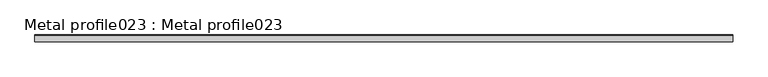
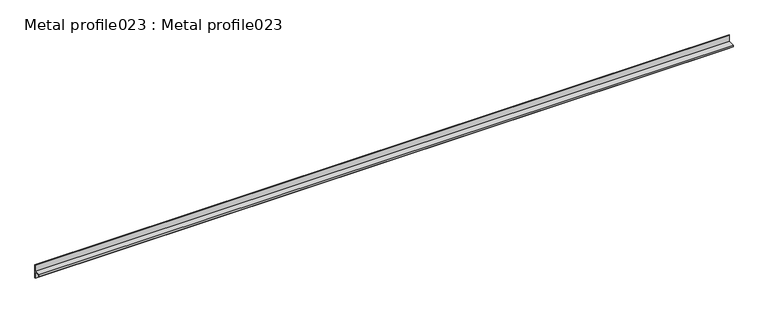
"""IFC4 building model written with IfcOpenShell, lengths in millimetres: proxy geometry, Metal profile023 : Metal profile023."""

from ifc_helpers import new_model, si_unit, frame, origin, place, context, project, spatial, polyline, outline, extrude, source, transform, mapped, element, save


def metal_profile023_metal_profile023_0d9bca16(model_context):
    return source(origin(), model_context, "Body", "SweptSolid", [
        extrude(outline(polyline([(-4684.6182816, 39724.0346875), (-4684.6182816, 39720.5548875), (-4685.8882816, 39720.5548875), (-4685.8882816, 39725.3046875), (-4667.6543336, 39725.3046875), (-4667.6543336, 39744.3546875), (-4666.3843336, 39744.3546875), (-4666.3843336, 39704.9846875), (-4667.6543336, 39704.9846875), (-4667.6543336, 39724.0346875), (-4684.6182816, 39724.0346875)])), frame((12383.0178845, 0.0, 0.0), z_axis=(1.0, 0.0, 0.0), x_axis=(0.0, 1.0, 0.0)), (0.0, 0.0, 1.0), 2000.0),
    ])


if __name__ == "__main__":
    model = new_model("IFC4")
    model_context = context("Model", 3, world=origin())
    ifc_project = project(units=[si_unit("LENGTHUNIT", "METRE", prefix="MILLI")], contexts=[model_context])
    site = spatial("IfcSite", under=ifc_project)
    building = spatial("IfcBuilding", under=site)
    placement = place(None, origin())
    metal_profile023_metal_profile023_shape = metal_profile023_metal_profile023_0d9bca16(model_context)
    element("IfcBuildingElementProxy", 1, Name="Metal profile023 : Metal profile023", ObjectType="Metal profile023 : Metal profile023", at=placement, inside=building, context=model_context, shape_type="MappedRepresentation", body=[
        mapped(metal_profile023_metal_profile023_shape, transform((0.0, 0.0, 0.0), x_axis=(1.0, 0.0, 0.0), y_axis=(0.0, 1.0, 0.0), z_axis=(0.0, 0.0, 1.0))),
    ])
    save(model, "model.ifc")

# Revit data of these elements
# Type "Metal profile023 : Metal profile023"
#   NameOverride = "Metal profile023"
# Element 1 (IfcBuildingElementProxy, "Metal profile023 : Metal profile023")
#   Materials on its faces: "16 GA. COPPER VENTED T REVEAL BEAD"
# Materials
#   "16 GA. COPPER VENTED T REVEAL BEAD": class "Unassigned", colour RGB 255 227 10, transparency 0
